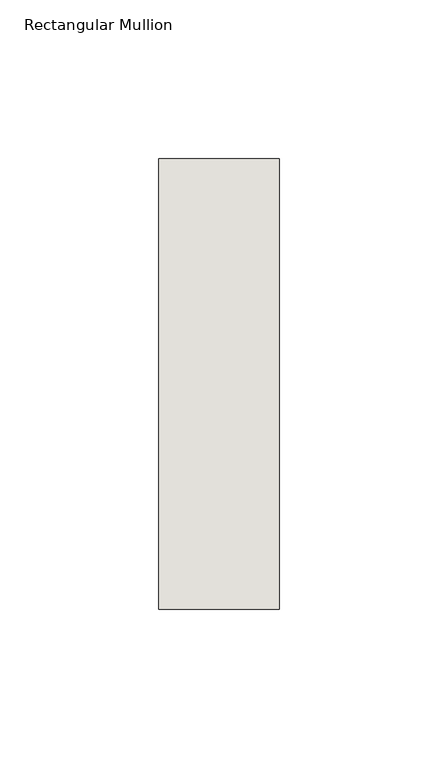
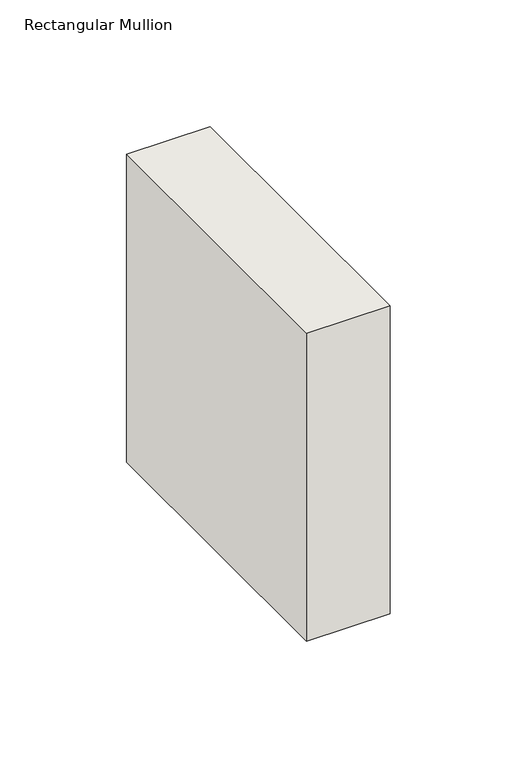
"""IFC4 building model written with IfcOpenShell, lengths in millimetres: wall geometry, Rectangular Mullion : NLRS_21_CWM_hsb-regel 38x142_gen_rsf."""

from ifc_helpers import new_model, si_unit, frame, origin, place, context, project, spatial, polyline, outline, extrude, source, transform, mapped, element, save


def rectangular_mullion_8a963fb8(model_context):
    return source(origin(), model_context, "Body", "SweptSolid", [
        extrude(outline(polyline([(19.0, -71.0), (-19.0, -71.0), (-19.0, 71.0), (19.0, 71.0), (19.0, -71.0)])), frame((0.0, 0.0, -148.1558939), z_axis=(0.0, 0.0, 1.0), x_axis=(1.0, 0.0, 0.0)), (0.0, 0.0, 1.0), 148.1558939),
    ])


if __name__ == "__main__":
    model = new_model("IFC4")
    model_context = context("Model", 3, world=origin())
    ifc_project = project(units=[si_unit("LENGTHUNIT", "METRE", prefix="MILLI")], contexts=[model_context])
    site = spatial("IfcSite", under=ifc_project)
    building = spatial("IfcBuilding", under=site)
    placement = place(None, origin())
    rectangular_mullion_shape = rectangular_mullion_8a963fb8(model_context)
    element("IfcWall", 1, ObjectType="Rectangular Mullion : NLRS_21_CWM_hsb-regel 38x142_gen_rsf", at=placement, inside=building, context=model_context, shape_type="MappedRepresentation", body=[
        mapped(rectangular_mullion_shape, transform((0.0, 0.0, 0.0), x_axis=(1.0, 0.0, 0.0), y_axis=(0.0, 1.0, 0.0), z_axis=(0.0, 0.0, 1.0))),
    ])
    save(model, "model.ifc")

# Revit data of these elements
# Type "Rectangular Mullion : NLRS_21_CWM_hsb-regel 38x142_gen_rsf"
#   Type IfcGUID = "07M7mRoiH1CR8m_RSKIwpF"
#   Assembly Code = "21.10"
#   IfcExportAs = "IfcWall"
#   built-in parameter 1007322 = 0.465879 (stored number, unit not read)
#   built-in parameter 1007321 = 0.062336 (stored number, unit not read)
#   built-in parameter 1007320 = 0.062336 (stored number, unit not read)
# Element 1 (IfcWall, "Rectangular Mullion : NLRS_21_CWM_hsb-regel 38x142_gen_rsf")
#   Materials on its faces: "NLRS_i2_hout naaldhout vuren_gen_rsf"
# Materials
#   "NLRS_i2_hout naaldhout vuren_gen_rsf": class "I - Hout", colour RGB 234 199 147, transparency 0, Keynote = "i2", Manufacturer = "Revit Standards Foundation", URL = "www.revitstandards.org", Description = "hout vuren", Cost = 0
